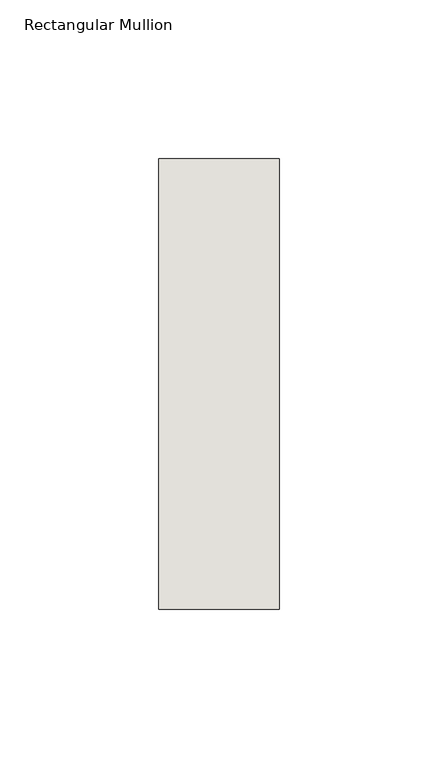
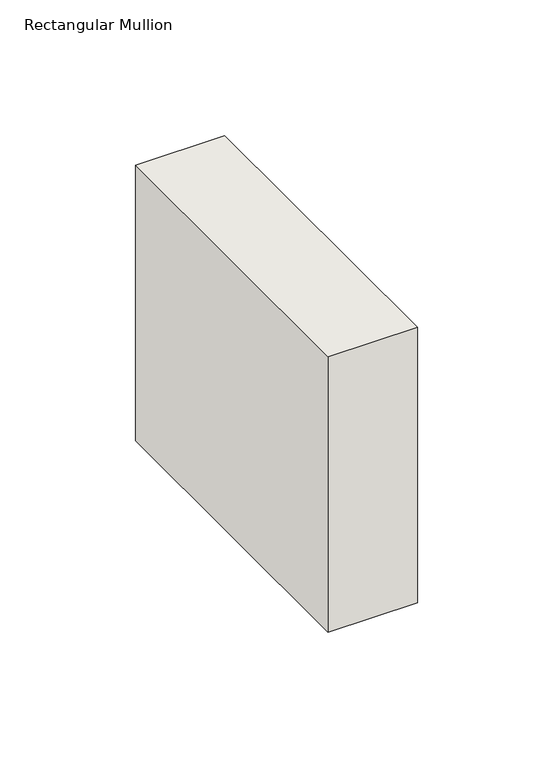
"""IFC4 building model written with IfcOpenShell, lengths in millimetres: wall geometry, Rectangular Mullion : NLRS_21_CWM_hsb-regel 38x142_gen_rsf."""

from ifc_helpers import new_model, si_unit, frame, origin, place, context, project, spatial, polyline, outline, extrude, source, transform, mapped, element, save


def rectangular_mullion_0b08a0e2(model_context):
    return source(origin(), model_context, "Body", "SweptSolid", [
        extrude(outline(polyline([(0.0, -71.0), (-38.0, -71.0), (-38.0, 71.0), (0.0, 71.0), (0.0, -71.0)])), frame((0.0, 0.0, -123.9999997), z_axis=(0.0, 0.0, 1.0), x_axis=(1.0, 0.0, 0.0)), (0.0, 0.0, 1.0), 123.9999997),
    ])


if __name__ == "__main__":
    model = new_model("IFC4")
    model_context = context("Model", 3, world=origin())
    ifc_project = project(units=[si_unit("LENGTHUNIT", "METRE", prefix="MILLI")], contexts=[model_context])
    site = spatial("IfcSite", under=ifc_project)
    building = spatial("IfcBuilding", under=site)
    placement = place(None, origin())
    rectangular_mullion_shape = rectangular_mullion_0b08a0e2(model_context)
    element("IfcWall", 1, ObjectType="Rectangular Mullion : NLRS_21_CWM_hsb-regel 38x142_gen_rsf", at=placement, inside=building, context=model_context, shape_type="MappedRepresentation", body=[
        mapped(rectangular_mullion_shape, transform((0.0, 0.0, 0.0), x_axis=(1.0, 0.0, 0.0), y_axis=(0.0, 1.0, 0.0), z_axis=(0.0, 0.0, 1.0))),
    ])
    save(model, "model.ifc")

# Revit data of these elements
# Type "Rectangular Mullion : NLRS_21_CWM_hsb-regel 38x142_gen_rsf"
#   Type IfcGUID = "07M7mRoiH1CR8m_RSKIwpF"
#   Assembly Code = "21.10"
#   IfcExportAs = "IfcWall"
#   built-in parameter 1007322 = 0.465879 (stored number, unit not read)
#   built-in parameter 1007321 = 0.062336 (stored number, unit not read)
#   built-in parameter 1007320 = 0.062336 (stored number, unit not read)
# Element 1 (IfcWall, "Rectangular Mullion : NLRS_21_CWM_hsb-regel 38x142_gen_rsf")
#   Materials on its faces: "NLRS_i2_hout naaldhout vuren_gen_rsf"
# Materials
#   "NLRS_i2_hout naaldhout vuren_gen_rsf": class "I - Hout", colour RGB 234 199 147, transparency 0, Keynote = "i2", Manufacturer = "Revit Standards Foundation", URL = "www.revitstandards.org", Description = "hout vuren", Cost = 0
